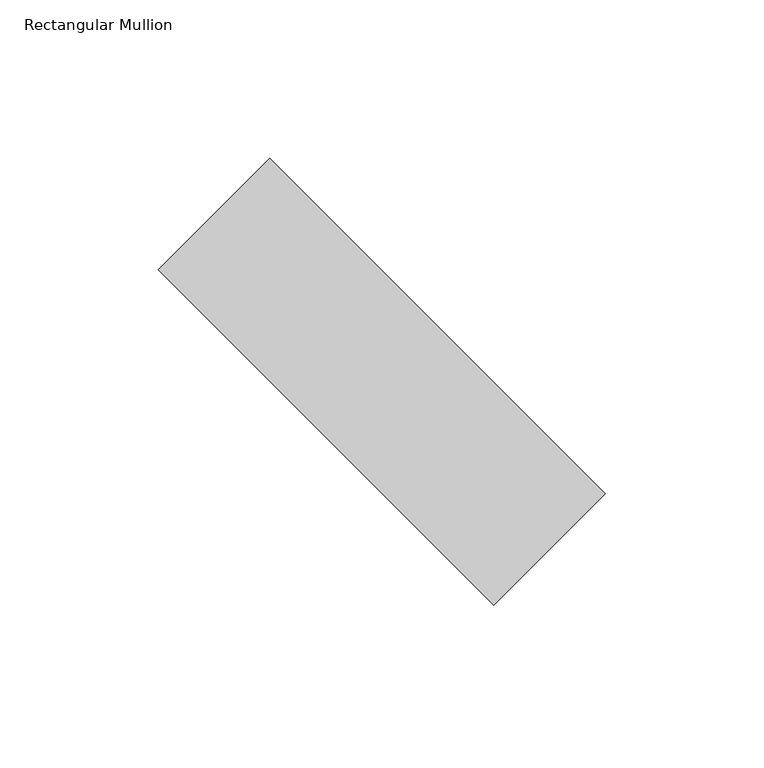
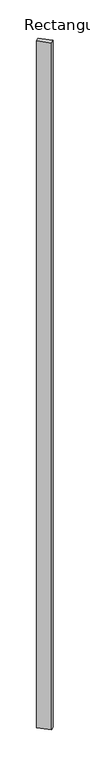
"""IFC4 building model written with IfcOpenShell, lengths in millimetres: member geometry, Rectangular Mullion : tilted mullions."""

from ifc_helpers import new_model, si_unit, frame, origin, place, context, project, spatial, polyline, outline, extrude, source, transform, mapped, element, save


def rectangular_mullion_42344c31(model_context):
    return source(origin(), model_context, "Body", "SweptSolid", [
        extrude(outline(polyline([(-35.3553391, 70.7106781), (70.7106781, -35.3553391), (35.3553391, -70.7106781), (-70.7106781, 35.3553391), (-35.3553391, 70.7106781)])), frame((0.0, 0.0, -7999.2546449), z_axis=(0.0, 0.0, 1.0), x_axis=(1.0, 0.0, 0.0)), (0.0, 0.0, 1.0), 7999.2546449),
    ])


if __name__ == "__main__":
    model = new_model("IFC4")
    model_context = context("Model", 3, world=origin())
    ifc_project = project(units=[si_unit("LENGTHUNIT", "METRE", prefix="MILLI")], contexts=[model_context])
    site = spatial("IfcSite", under=ifc_project)
    building = spatial("IfcBuilding", under=site)
    placement = place(None, origin())
    rectangular_mullion_shape = rectangular_mullion_42344c31(model_context)
    element("IfcMember", 1, ObjectType="Rectangular Mullion : tilted mullions", at=placement, inside=building, context=model_context, shape_type="MappedRepresentation", body=[
        mapped(rectangular_mullion_shape, transform((0.0, 0.0, 0.0), x_axis=(1.0, 0.0, 0.0), y_axis=(0.0, 1.0, 0.0), z_axis=(0.0, 0.0, 1.0))),
    ])
    save(model, "model.ifc")

# Revit data of these elements
# Type "Rectangular Mullion : tilted mullions"
#   built-in parameter 1007304 = 0.492126 (stored number, unit not read)
#   built-in parameter 1007301 = 0.082021 (stored number, unit not read)
#   built-in parameter 1007300 = 0.082021 (stored number, unit not read)
# Element 1 (IfcMember, "Rectangular Mullion : tilted mullions")
#   Materials on its faces: "Aluminum"
# Materials
#   "Aluminum": class "Metal", colour RGB 244 244 244, transparency 0, Description = "Aluminum 6061", Cost = 0
